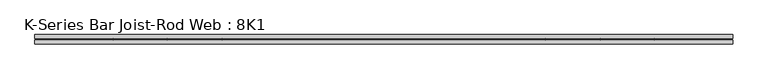
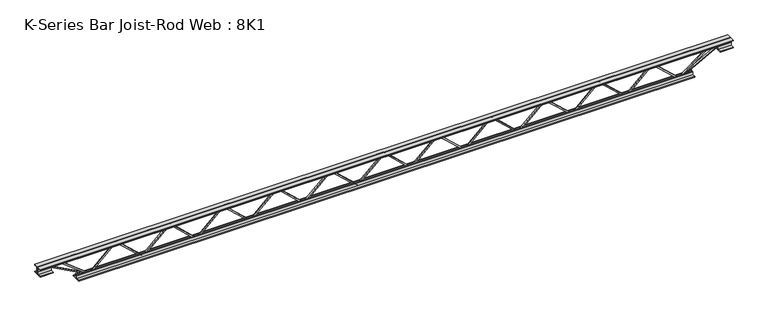
"""IFC4 building model written with IfcOpenShell, lengths in millimetres: beam geometry, K-Series Bar Joist-Rod Web : 8K1."""

from ifc_helpers import new_model, si_unit, frame, origin, place, context, project, spatial, polyline, outline, extrude, source, transform, mapped, element, save


def k_series_bar_joist_rod_web_8k1_abf054b3(model_context):
    return source(origin(), model_context, "Body", "SweptSolid", [
        extrude(outline(polyline([(-90.4875, 1487.0545455), (-100.0125, 1487.0545455), (-100.0125, 1492.0935213), (90.4875, 1698.1798849), (90.4875, 1700.8019332), (-100.0125, 1906.8882969), (-100.0125, 1911.9272727), (-90.4875, 1911.9272727), (-90.4875, 1910.6162486), (100.0125, 1704.5298849), (100.0125, 1694.4519332), (-90.4875, 1488.3655696), (-90.4875, 1487.0545455)])), frame((0.0, -4.7625, 0.0), z_axis=(0.0, 1.0, 0.0), x_axis=(0.0, 0.0, 1.0)), (0.0, 0.0, 1.0), 9.525),
        extrude(outline(polyline([(-90.4875, 1062.1818182), (-100.0125, 1062.1818182), (-100.0125, 1067.220794), (90.4875, 1273.3071577), (90.4875, 1275.929206), (-100.0125, 1482.0155696), (-100.0125, 1487.0545455), (-90.4875, 1487.0545455), (-90.4875, 1485.7435213), (100.0125, 1279.6571577), (100.0125, 1269.579206), (-90.4875, 1063.4928423), (-90.4875, 1062.1818182)])), frame((0.0, -4.7625, 0.0), z_axis=(0.0, 1.0, 0.0), x_axis=(0.0, 0.0, 1.0)), (0.0, 0.0, 1.0), 9.525),
        extrude(outline(polyline([(-90.4875, 637.3090909), (-100.0125, 637.3090909), (-100.0125, 642.3480668), (90.4875, 848.4344304), (90.4875, 851.0564787), (-100.0125, 1057.1428423), (-100.0125, 1062.1818182), (-90.4875, 1062.1818182), (-90.4875, 1060.870794), (100.0125, 854.7844304), (100.0125, 844.7064787), (-90.4875, 638.6201151), (-90.4875, 637.3090909)])), frame((0.0, -4.7625, 0.0), z_axis=(0.0, 1.0, 0.0), x_axis=(0.0, 0.0, 1.0)), (0.0, 0.0, 1.0), 9.525),
        extrude(outline(polyline([(-90.4875, 212.4363636), (-100.0125, 212.4363636), (-100.0125, 217.4753395), (90.4875, 423.5617031), (90.4875, 426.1837514), (-100.0125, 632.2701151), (-100.0125, 637.3090909), (-90.4875, 637.3090909), (-90.4875, 635.9980668), (100.0125, 429.9117031), (100.0125, 419.8337514), (-90.4875, 213.7473878), (-90.4875, 212.4363636)])), frame((0.0, -4.7625, 0.0), z_axis=(0.0, 1.0, 0.0), x_axis=(0.0, 0.0, 1.0)), (0.0, 0.0, 1.0), 9.525),
        extrude(outline(polyline([(-90.4875, -212.4363636), (-100.0125, -212.4363636), (-100.0125, -207.3973878), (90.4875, -1.3110241), (90.4875, 1.3110241), (-100.0125, 207.3973878), (-100.0125, 212.4363636), (-90.4875, 212.4363636), (-90.4875, 211.1253395), (100.0125, 5.0389759), (100.0125, -5.0389759), (-90.4875, -211.1253395), (-90.4875, -212.4363636)])), frame((0.0, -4.7625, 0.0), z_axis=(0.0, 1.0, 0.0), x_axis=(0.0, 0.0, 1.0)), (0.0, 0.0, 1.0), 9.525),
        extrude(outline(polyline([(-90.4875, -637.3090909), (-100.0125, -637.3090909), (-100.0125, -632.2701151), (90.4875, -426.1837514), (90.4875, -423.5617031), (-100.0125, -217.4753395), (-100.0125, -212.4363636), (-90.4875, -212.4363636), (-90.4875, -213.7473878), (100.0125, -419.8337514), (100.0125, -429.9117031), (-90.4875, -635.9980668), (-90.4875, -637.3090909)])), frame((0.0, -4.7625, 0.0), z_axis=(0.0, 1.0, 0.0), x_axis=(0.0, 0.0, 1.0)), (0.0, 0.0, 1.0), 9.525),
        extrude(outline(polyline([(-90.4875, -1062.1818182), (-100.0125, -1062.1818182), (-100.0125, -1057.1428423), (90.4875, -851.0564787), (90.4875, -848.4344304), (-100.0125, -642.3480668), (-100.0125, -637.3090909), (-90.4875, -637.3090909), (-90.4875, -638.6201151), (100.0125, -844.7064787), (100.0125, -854.7844304), (-90.4875, -1060.870794), (-90.4875, -1062.1818182)])), frame((0.0, -4.7625, 0.0), z_axis=(0.0, 1.0, 0.0), x_axis=(0.0, 0.0, 1.0)), (0.0, 0.0, 1.0), 9.525),
        extrude(outline(polyline([(-90.4875, -1487.0545455), (-100.0125, -1487.0545455), (-100.0125, -1482.0155696), (90.4875, -1275.929206), (90.4875, -1273.3071577), (-100.0125, -1067.220794), (-100.0125, -1062.1818182), (-90.4875, -1062.1818182), (-90.4875, -1063.4928423), (100.0125, -1269.579206), (100.0125, -1279.6571577), (-90.4875, -1485.7435213), (-90.4875, -1487.0545455)])), frame((0.0, -4.7625, 0.0), z_axis=(0.0, 1.0, 0.0), x_axis=(0.0, 0.0, 1.0)), (0.0, 0.0, 1.0), 9.525),
        extrude(outline(polyline([(-90.4875, -1911.9272727), (-100.0125, -1911.9272727), (-100.0125, -1906.8882969), (90.4875, -1700.8019332), (90.4875, -1698.1798849), (-100.0125, -1492.0935213), (-100.0125, -1487.0545455), (-90.4875, -1487.0545455), (-90.4875, -1488.3655696), (100.0125, -1694.4519332), (100.0125, -1704.5298849), (-90.4875, -1910.6162486), (-90.4875, -1911.9272727)])), frame((0.0, -4.7625, 0.0), z_axis=(0.0, 1.0, 0.0), x_axis=(0.0, 0.0, 1.0)), (0.0, 0.0, 1.0), 9.525),
        extrude(outline(polyline([(-90.4875, 1911.9272727), (-100.0125, 1911.9272727), (-100.0125, 1916.9662486), (90.4875, 2123.0526122), (90.4875, 2125.6746605), (-100.0125, 2331.7610241), (-100.0125, 2336.8), (-90.4875, 2336.8), (-90.4875, 2335.4889759), (100.0125, 2129.4026122), (100.0125, 2119.3246605), (-90.4875, 1913.2382969), (-90.4875, 1911.9272727)])), frame((0.0, -4.7625, 0.0), z_axis=(0.0, 1.0, 0.0), x_axis=(0.0, 0.0, 1.0)), (0.0, 0.0, 1.0), 9.525),
        extrude(outline(polyline([(-90.4875, -2336.8), (-100.0125, -2336.8), (-100.0125, -2331.7610241), (90.4875, -2125.6746605), (90.4875, -2123.0526122), (-100.0125, -1916.9662486), (-100.0125, -1911.9272727), (-90.4875, -1911.9272727), (-90.4875, -1913.2382969), (100.0125, -2119.3246605), (100.0125, -2129.4026122), (-90.4875, -2335.4889759), (-90.4875, -2336.8)])), frame((0.0, -4.7625, 0.0), z_axis=(0.0, 1.0, 0.0), x_axis=(0.0, 0.0, 1.0)), (0.0, 0.0, 1.0), 9.525),
        extrude(outline(polyline([(4.7625, 101.6), (36.5125, 101.6), (36.5125, 95.25), (11.1125, 95.25), (11.1125, 69.85), (4.7625, 69.85), (4.7625, 101.6)])), frame((-2743.2, 0.0, 0.0), z_axis=(1.0, 0.0, 0.0), x_axis=(0.0, 1.0, 0.0)), (0.0, 0.0, 1.0), 5486.4),
        extrude(outline(polyline([(-4.7625, 101.6), (-4.7625, 69.85), (-11.1125, 69.85), (-11.1125, 95.25), (-36.5125, 95.25), (-36.5125, 101.6), (-4.7625, 101.6)])), frame((-2743.2, 0.0, 0.0), z_axis=(1.0, 0.0, 0.0), x_axis=(0.0, 1.0, 0.0)), (0.0, 0.0, 1.0), 5486.4),
        extrude(outline(polyline([(-4.7625, 38.1), (-36.5125, 38.1), (-36.5125, 44.45), (-11.1125, 44.45), (-11.1125, 69.85), (-4.7625, 69.85), (-4.7625, 38.1)])), frame((-2743.2, 0.0, 0.0), z_axis=(1.0, 0.0, 0.0), x_axis=(0.0, 1.0, 0.0)), (0.0, 0.0, 1.0), 101.6),
        extrude(outline(polyline([(36.5125, 38.1), (4.7625, 38.1), (4.7625, 69.85), (11.1125, 69.85), (11.1125, 44.45), (36.5125, 44.45), (36.5125, 38.1)])), frame((-2743.2, 0.0, 0.0), z_axis=(1.0, 0.0, 0.0), x_axis=(0.0, 1.0, 0.0)), (0.0, 0.0, 1.0), 101.6),
        extrude(outline(polyline([(4.7625, 38.1), (4.7625, 69.85), (11.1125, 69.85), (11.1125, 44.45), (36.5125, 44.45), (36.5125, 38.1), (4.7625, 38.1)])), frame((2641.6, 0.0, 0.0), z_axis=(1.0, 0.0, 0.0), x_axis=(0.0, 1.0, 0.0)), (0.0, 0.0, 1.0), 101.6),
        extrude(outline(polyline([(-4.7625, 38.1), (-36.5125, 38.1), (-36.5125, 44.45), (-11.1125, 44.45), (-11.1125, 69.85), (-4.7625, 69.85), (-4.7625, 38.1)])), frame((2641.6, 0.0, 0.0), z_axis=(1.0, 0.0, 0.0), x_axis=(0.0, 1.0, 0.0)), (0.0, 0.0, 1.0), 101.6),
        extrude(outline(polyline([(4.7625, -101.6), (4.7625, -69.85), (11.1125, -69.85), (11.1125, -95.25), (36.5125, -95.25), (36.5125, -101.6), (4.7625, -101.6)])), frame((-2438.4, 0.0, 0.0), z_axis=(1.0, 0.0, 0.0), x_axis=(0.0, 1.0, 0.0)), (0.0, 0.0, 1.0), 4876.8),
        extrude(outline(polyline([(-4.7625, -101.6), (-36.5125, -101.6), (-36.5125, -95.25), (-11.1125, -95.25), (-11.1125, -69.85), (-4.7625, -69.85), (-4.7625, -101.6)])), frame((-2438.4, 0.0, 0.0), z_axis=(1.0, 0.0, 0.0), x_axis=(0.0, 1.0, 0.0)), (0.0, 0.0, 1.0), 4876.8),
        extrude(outline(polyline([(0.0, -9.525), (0.0, 0.0), (346.6425392, 0.0), (346.6425392, -9.525), (0.0, -9.525)])), frame((-2643.8682985, 4.7625, 65.662372), z_axis=(0.47628314854007986, 0.0, 0.8792919665371386), x_axis=(0.8792919665371386, 0.0, -0.47628314854007986)), (0.0, 0.0, 1.0), 9.525),
        extrude(outline(polyline([(0.0, -9.525), (0.0, 0.0), (269.048729, 0.0), (269.048729, -9.525), (0.0, -9.525)])), frame((-2552.1588407, 4.7625, 66.0896099), z_axis=(0.6136434860418419, 0.0, 0.7895832267965269), x_axis=(0.7895832267965269, 0.0, -0.6136434860418419)), (0.0, 0.0, 1.0), 9.525),
        extrude(outline(polyline([(0.0, -9.525), (0.0, 0.0), (346.6425392, 0.0), (346.6425392, -9.525), (0.0, -9.525)])), frame((2643.8682985, -4.7625, 65.662372), z_axis=(-0.4762831485400416, 0.0, 0.8792919665371592), x_axis=(-0.8792919665371592, 0.0, -0.4762831485400416)), (0.0, 0.0, 1.0), 9.525),
        extrude(outline(polyline([(0.0, -9.525), (0.0, 0.0), (269.048729, 0.0), (269.048729, -9.525), (0.0, -9.525)])), frame((2552.1588407, -4.7625, 66.0896099), z_axis=(-0.6136434860418192, 0.0, 0.7895832267965447), x_axis=(-0.7895832267965447, 0.0, -0.6136434860418192)), (0.0, 0.0, 1.0), 9.525),
    ])


if __name__ == "__main__":
    model = new_model("IFC4")
    model_context = context("Model", 3, world=origin())
    ifc_project = project(units=[si_unit("LENGTHUNIT", "METRE", prefix="MILLI")], contexts=[model_context])
    site = spatial("IfcSite", under=ifc_project)
    building = spatial("IfcBuilding", under=site)
    placement = place(None, origin())
    k_series_bar_joist_rod_web_8k1_shape = k_series_bar_joist_rod_web_8k1_abf054b3(model_context)
    element("IfcBeam", 1, ObjectType="K-Series Bar Joist-Rod Web : 8K1", at=placement, inside=building, context=model_context, shape_type="MappedRepresentation", body=[
        mapped(k_series_bar_joist_rod_web_8k1_shape, transform((0.0, 0.0, 0.0), x_axis=(1.0, 0.0, 0.0), y_axis=(0.0, 1.0, 0.0), z_axis=(0.0, 0.0, 1.0))),
    ])
    save(model, "model.ifc")

# Revit data of these elements
# Type "K-Series Bar Joist-Rod Web : 8K1"
#   Assembly Code = "B1010350"
#   Wt = 5.1
#   Web Thickness = 0' - 0 3/8"
#   Start Offset [instance default] = 0' - 0"
#   Start Extension [instance default] = 0' - 0"
#   Seat Length = 0' - 4"
#   Seat Depth = 0' - 2 1/2"
#   PanelArrayLength [instance default] = 21' - 4"
#   Panel [instance default] = 1' - 4"
#   End Offset [instance default] = 0' - 0"
#   End Extension [instance default] = 0' - 0"
#   End Panel = 1' - 4"
#   Cord Leg = 0' - 1 1/4"
#   Chord Thickness = 0' - 0 1/4"
#   Length [instance default] = 24' - 0"
#   Depth = 0' - 8"
#   PanelArrayNum [instance default] = 16
#   Rendering Material = none
# Element 1 (IfcBeam, "K-Series Bar Joist-Rod Web : 8K1")
#   PanelArrayLength = 15' - 4"
#   Panel = 1' - 4.72727"
#   PanelArrayNum = 11
